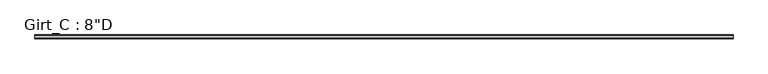
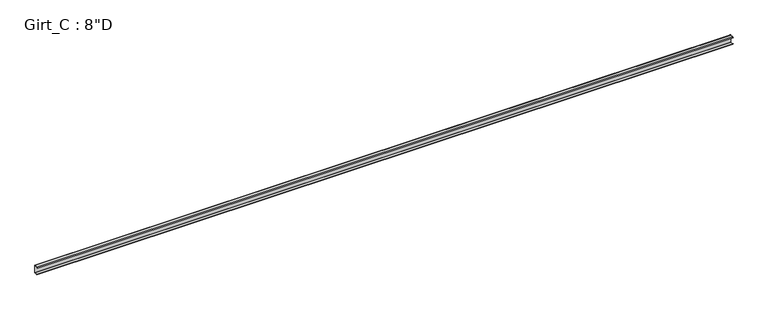
"""IFC4 building model written with IfcOpenShell, lengths in millimetres: beam geometry."""

from ifc_helpers import new_model, si_unit, point, frame, frame_2d, origin, place, context, project, spatial, polyline, circle_curve, trimmed, segment, composite_curve, outline, extrude, source, transform, mapped, element, save


def beam_41ea4732(model_context):
    return source(origin(), model_context, "Body", "SweptSolid", [
        extrude(outline(composite_curve([segment(polyline([(-87.5109375, 101.6), (-3.3734375, 101.6)]), True, "CONTINUOUS"), segment(trimmed(circle_curve(frame_2d((-3.3734375, 96.8375)), 4.7625), [point((-3.3734375, 101.6))], [point((1.3890625, 96.8375))], False, "CARTESIAN"), True, "CONTINUOUS"), segment(polyline([(1.3890625, 96.8375), (1.3890625, -96.8375)]), True, "CONTINUOUS"), segment(trimmed(circle_curve(frame_2d((-3.3734375, -96.8375)), 4.7625), [point((1.3890625, -96.8375))], [point((-3.3734375, -101.6))], False, "CARTESIAN"), True, "CONTINUOUS"), segment(polyline([(-3.3734375, -101.6), (-87.5109375, -101.6), (-99.7792647, -86.979177), (-97.6510975, -85.1934327), (-86.2154765, -98.821875), (-3.2694106, -98.821875)]), True, "CONTINUOUS"), segment(trimmed(circle_curve(frame_2d((-3.3748024, -96.8389339)), 1.9857399), [point((-3.2694106, -98.821875))], [point((-1.3890625, -96.8389339))], True, "CARTESIAN"), True, "CONTINUOUS"), segment(polyline([(-1.3890625, -96.8389339), (-1.3890625, 96.8381931)]), True, "CONTINUOUS"), segment(trimmed(circle_curve(frame_2d((-3.3741066, 96.8381931)), 1.9850441), [point((-1.3890625, 96.8381931))], [point((-3.3005807, 98.821875))], True, "CARTESIAN"), True, "CONTINUOUS"), segment(polyline([(-3.3005807, 98.821875), (-86.2154765, 98.821875), (-97.6278742, 85.221109), (-99.7560415, 87.0068534), (-87.5109375, 101.6)]), True, "CONTINUOUS")], self_intersect=False)), frame((-9088.3762054, 0.0, 0.0), z_axis=(1.0, 0.0, 0.0), x_axis=(0.0, 1.0, 0.0)), (0.0, 0.0, 1.0), 18176.7524108),
    ])


if __name__ == "__main__":
    model = new_model("IFC4")
    model_context = context("Model", 3, world=origin())
    ifc_project = project(units=[si_unit("LENGTHUNIT", "METRE", prefix="MILLI")], contexts=[model_context])
    site = spatial("IfcSite", under=ifc_project)
    building = spatial("IfcBuilding", under=site)
    placement = place(None, origin())
    beam_shape = beam_41ea4732(model_context)
    element("IfcBeam", 1, ObjectType="Girt_C : 8\"D", at=placement, inside=building, context=model_context, shape_type="MappedRepresentation", body=[
        mapped(beam_shape, transform((0.0, 0.0, 0.0), x_axis=(1.0, 0.0, 0.0), y_axis=(0.0, 1.0, 0.0), z_axis=(0.0, 0.0, 1.0))),
    ])
    save(model, "model.ifc")

# Revit data of these elements
# Type "Girt_C : 8\"D"
#   half leg = 0' - 1 3/4"
#   Web_Thickness = 0' - 0 7/64"
#   Length [instance default] = 10' - 0"
#   Leg_1 = 0' - 3 1/2"
#   Height = 0' - 8"
#   Structural Material [instance default] = none
# Element 1 (IfcBeam, "Girt_C : 8\"D")
#   Structural Material = CEE' SECTION (8.0x3.5C - SEE STRUCT. DWGS)
#   Materials on its faces: "CEE' SECTION (8.0x3.5C - SEE STRUCT. DWGS)"
# Materials
#   "CEE' SECTION (8.0x3.5C - SEE STRUCT. DWGS)": class "Metal", colour RGB 137 146 153, transparency 0, Description = "Steel, mill finish", Cost = 0
